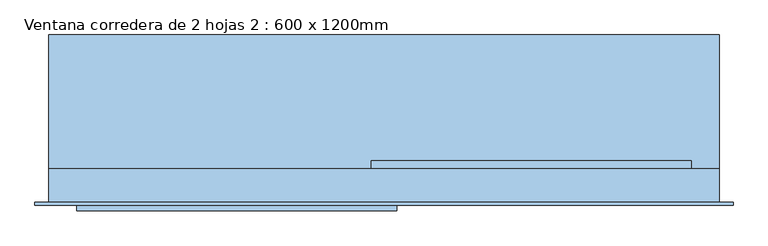
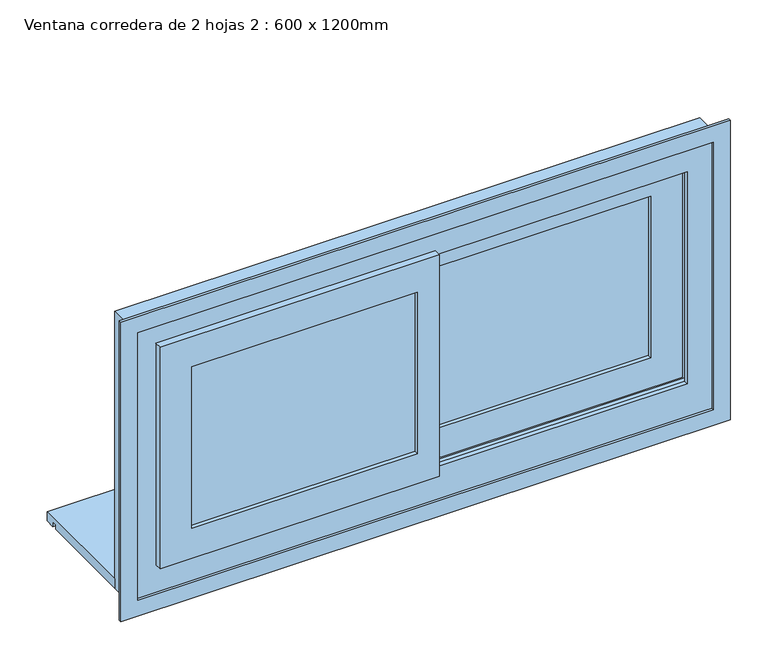
"""IFC4 building model written with IfcOpenShell, lengths in millimetres: window geometry, Ventana corredera de 2 hojas 2 : 600 x 1200mm."""

from ifc_helpers import new_model, si_unit, frame, origin, place, context, project, spatial, polyline, outline, extrude, faceted_brep, source, transform, mapped, element, save


def ventana_corredera_de_2_hojas_2_600_x_1200mm_91e0f78e(model_context):
    return source(origin(), model_context, "Body", "SolidModel", [
        extrude(outline(polyline([(225.0, 920.0), (225.0, 900.0), (205.0, 900.0), (205.0, 910.0), (195.0, 910.0), (195.0, 900.0), (-15.0, 900.0), (-15.0, 920.0), (225.0, 920.0)])), frame((-600.0, 0.0, 0.0), z_axis=(1.0, 0.0, 0.0), x_axis=(0.0, 1.0, 0.0)), (0.0, 0.0, 1.0), 1200.0),
        faceted_brep([(22.5, -90.0, 970.0011599), (22.5, -75.0, 970.0011599), (22.5, -75.0, 990.0011599), (22.5, -65.0, 990.0011599), (22.5, -65.0, 970.0011599), (22.5, -42.0, 970.0011599), (22.5, -42.0, 1449.9988401), (22.5, -65.0, 1449.9988401), (22.5, -65.0, 1429.9988401), (22.5, -75.0, 1429.9988401), (22.5, -75.0, 1449.9988401), (22.5, -90.0, 1449.9988401), (-549.9988401, -90.0, 970.0011599), (-549.9988401, -75.0, 970.0011599), (-549.9988401, -75.0, 1449.9988401), (-529.9988401, -75.0, 1429.9988401), (-529.9988401, -75.0, 990.0011599), (-529.9988401, -65.0, 990.0011599), (-529.9988401, -65.0, 1429.9988401), (-549.9988401, -65.0, 1449.9988401), (-549.9988401, -65.0, 970.0011599), (-549.9988401, -50.0, 970.0011599), (0.0, -50.0, 970.0011599), (0.0, -42.0, 970.0011599), (0.0, -42.0, 1449.9988401), (-549.9988401, -90.0, 1449.9988401), (-484.9988401, -90.0, 1035.0011599), (-484.9988401, -90.0, 1384.9988401), (-22.5, -90.0, 1384.9988401), (-22.5, -90.0, 1035.0011599), (-549.9988401, -50.0, 1449.9988401), (0.0, -50.0, 1449.9988401), (-484.9988401, -50.0, 1384.9988401), (-484.9988401, -50.0, 1035.0011599), (-22.5, -50.0, 1035.0011599), (-22.5, -50.0, 1384.9988401), (-484.9988401, -58.0, 1384.9988401), (-484.9988401, -58.0, 1035.0011599), (-22.5, -58.0, 1035.0011599), (-22.5, -58.0, 1384.9988401), (-484.9988401, -82.0, 1035.0011599), (-484.9988401, -82.0, 1384.9988401), (-22.5, -82.0, 1384.9988401), (-22.5, -82.0, 1035.0011599), (-504.9988401, -82.0, 1015.0011599), (-504.9988401, -82.0, 1404.9988401), (-2.5, -82.0, 1404.9988401), (-2.5, -82.0, 1015.0011599), (-504.9988401, -58.0, 1015.0011599), (-504.9988401, -58.0, 1404.9988401), (-2.5, -58.0, 1015.0011599), (-2.5, -58.0, 1404.9988401)], [[[0, 1, 2, 3, 4, 5, 6, 7, 8, 9, 10, 11]], [[1, 0, 12, 13]], [[2, 1, 13, 14, 10, 9, 15, 16]], [[3, 2, 16, 17]], [[4, 3, 17, 18, 8, 7, 19, 20]], [[5, 4, 20, 21, 22, 23]], [[6, 5, 23, 24]], [[12, 0, 11, 25], [26, 27, 28, 29]], [[21, 30, 31, 22], [32, 33, 34, 35]], [[30, 21, 20, 19]], [[24, 23, 22, 31]], [[33, 32, 36, 37]], [[33, 37, 38, 34]], [[38, 39, 35, 34]], [[18, 17, 16, 15]], [[14, 13, 12, 25]], [[27, 26, 40, 41]], [[29, 28, 42, 43]], [[40, 26, 29, 43]], [[44, 45, 46, 47], [41, 40, 43, 42]], [[45, 44, 48, 49]], [[50, 47, 46, 51]], [[48, 44, 47, 50]], [[49, 48, 50, 51], [37, 36, 39, 38]], [[19, 7, 6, 24, 31, 30]], [[8, 18, 15, 9]], [[10, 14, 25, 11]], [[36, 32, 35, 39]], [[27, 41, 42, 28]], [[45, 49, 51, 46]]]),
        faceted_brep([(-22.5, 0.0, 1449.9988401), (549.9988401, 0.0, 1449.9988401), (549.9988401, 0.0, 970.0011599), (-22.5, 0.0, 970.0011599), (484.9988401, 0.0, 1035.0011599), (484.9988401, 0.0, 1384.9988401), (22.5, 0.0, 1384.9988401), (22.5, 0.0, 1035.0011599), (549.9988401, -15.0, 1449.9988401), (549.9988401, -15.0, 970.0011599), (-22.5, -15.0, 970.0011599), (-22.5, -25.0, 1449.9988401), (-22.5, -25.0, 1429.9988401), (-22.5, -15.0, 1429.9988401), (-22.5, -15.0, 1449.9988401), (-22.5, -15.0, 990.0011599), (-22.5, -25.0, 990.0011599), (-22.5, -25.0, 970.0011599), (-22.5, -48.0, 970.0011599), (-22.5, -48.0, 1449.9988401), (484.9988401, -8.0, 1035.0011599), (484.9988401, -8.0, 1384.9988401), (22.5, -8.0, 1384.9988401), (22.5, -8.0, 1035.0011599), (529.9988401, -15.0, 1429.9988401), (529.9988401, -15.0, 990.0011599), (529.9988401, -25.0, 990.0011599), (549.9988401, -25.0, 1449.9988401), (549.9988401, -25.0, 970.0011599), (529.9988401, -25.0, 1429.9988401), (549.9988401, -40.0, 970.0011599), (0.0, -40.0, 970.0011599), (0.0, -48.0, 970.0011599), (0.0, -48.0, 1449.9988401), (0.0, -40.0, 1449.9988401), (549.9988401, -40.0, 1449.9988401), (484.9988401, -40.0, 1384.9988401), (484.9988401, -40.0, 1035.0011599), (22.5, -40.0, 1035.0011599), (22.5, -40.0, 1384.9988401), (484.9988401, -32.0, 1384.9988401), (484.9988401, -32.0, 1035.0011599), (22.5, -32.0, 1035.0011599), (22.5, -32.0, 1384.9988401), (504.9988401, -32.0, 1404.9988401), (504.9988401, -32.0, 1015.0011599), (2.5, -32.0, 1015.0011599), (2.5, -32.0, 1404.9988401), (504.9988401, -8.0, 1404.9988401), (504.9988401, -8.0, 1015.0011599), (2.5, -8.0, 1015.0011599), (2.5, -8.0, 1404.9988401)], [[[0, 1, 2, 3], [4, 5, 6, 7]], [[8, 9, 2, 1]], [[9, 10, 3, 2]], [[11, 12, 13, 14, 0, 3, 10, 15, 16, 17, 18, 19]], [[5, 4, 20, 21]], [[7, 6, 22, 23]], [[20, 4, 7, 23]], [[14, 13, 24, 25, 15, 10, 9, 8]], [[26, 16, 15, 25]], [[12, 11, 27, 28, 17, 16, 26, 29]], [[18, 17, 28, 30, 31, 32]], [[19, 18, 32, 33]], [[33, 32, 31, 34]], [[30, 35, 34, 31], [36, 37, 38, 39]], [[37, 36, 40, 41]], [[37, 41, 42, 38]], [[39, 38, 42, 43]], [[35, 30, 28, 27]], [[44, 45, 46, 47], [41, 40, 43, 42]], [[48, 49, 45, 44]], [[45, 49, 50, 46]], [[51, 47, 46, 50]], [[49, 48, 51, 50], [21, 20, 23, 22]], [[29, 26, 25, 24]], [[0, 14, 8, 1]], [[5, 21, 22, 6]], [[13, 12, 29, 24]], [[11, 19, 33, 34, 35, 27]], [[40, 36, 39, 43]], [[48, 44, 47, 51]]]),
        extrude(outline(polyline([(-7.5, -58.0), (-7.5, -82.0), (-499.9988401, -82.0), (-499.9988401, -58.0), (-7.5, -58.0)])), frame((0.0, 0.0, 1020.0011599), z_axis=(0.0, 0.0, 1.0), x_axis=(1.0, 0.0, 0.0)), (0.0, 0.0, 1.0), 379.9976801),
        extrude(outline(polyline([(499.9988401, -8.0), (499.9988401, -32.0), (7.5, -32.0), (7.5, -8.0), (499.9988401, -8.0)])), frame((0.0, 0.0, 1020.0011599), z_axis=(0.0, 0.0, 1.0), x_axis=(1.0, 0.0, 0.0)), (0.0, 0.0, 1.0), 379.9976801),
        faceted_brep([(600.0, -15.0, 1500.0), (600.0, -75.0, 1500.0), (600.0, -75.0, 900.0), (600.0, -15.0, 900.0), (-600.0, -75.0, 1500.0), (-600.0, -75.0, 900.0), (-539.9988401, -75.0, 1439.9988401), (539.9988401, -75.0, 1439.9988401), (539.9988401, -75.0, 980.0011599), (-539.9988401, -75.0, 980.0011599), (-600.0, -15.0, 900.0), (-600.0, -15.0, 1500.0), (539.9988401, -15.0, 1439.9988401), (-539.9988401, -15.0, 1439.9988401), (-539.9988401, -15.0, 980.0011599), (539.9988401, -15.0, 980.0011599), (539.9988401, -25.0, 1439.9988401), (539.9988401, -25.0, 980.0011599), (-539.9988401, -25.0, 980.0011599), (564.9988401, -25.0, 1464.9988401), (-564.9988401, -25.0, 1464.9988401), (-564.9988401, -25.0, 955.0011599), (564.9988401, -25.0, 955.0011599), (-539.9988401, -25.0, 1439.9988401), (564.9988401, -65.0, 1464.9988401), (564.9988401, -65.0, 955.0011599), (-564.9988401, -65.0, 955.0011599), (-564.9988401, -65.0, 1464.9988401), (539.9988401, -65.0, 1439.9988401), (-539.9988401, -65.0, 1439.9988401), (-539.9988401, -65.0, 980.0011599), (539.9988401, -65.0, 980.0011599)], [[[0, 1, 2, 3]], [[2, 1, 4, 5], [6, 7, 8, 9]], [[3, 2, 5, 10]], [[10, 11, 0, 3], [12, 13, 14, 15]], [[16, 12, 15, 17]], [[17, 15, 14, 18]], [[19, 20, 21, 22], [23, 16, 17, 18]], [[24, 19, 22, 25]], [[25, 22, 21, 26]], [[27, 24, 25, 26], [28, 29, 30, 31]], [[7, 28, 31, 8]], [[8, 31, 30, 9]], [[13, 23, 18, 14]], [[20, 27, 26, 21]], [[29, 6, 9, 30]], [[4, 11, 10, 5]], [[11, 4, 1, 0]], [[23, 13, 12, 16]], [[27, 20, 19, 24]], [[6, 29, 28, 7]]]),
        extrude(outline(polyline([(1525.0, -625.0), (875.0, -625.0), (875.0, 625.0), (1525.0, 625.0), (1525.0, -625.0)]), holes=[polyline([(1490.0, 590.0), (910.0, 590.0), (910.0, -590.0), (1490.0, -590.0), (1490.0, 590.0)])]), frame((0.0, -80.0, 0.0), z_axis=(0.0, 1.0, 0.0), x_axis=(0.0, 0.0, 1.0)), (0.0, 0.0, 1.0), 5.0),
    ])


if __name__ == "__main__":
    model = new_model("IFC4")
    model_context = context("Model", 3, world=origin())
    ifc_project = project(units=[si_unit("LENGTHUNIT", "METRE", prefix="MILLI")], contexts=[model_context])
    site = spatial("IfcSite", under=ifc_project)
    building = spatial("IfcBuilding", under=site)
    placement = place(None, origin())
    ventana_corredera_de_2_hojas_2_600_x_1200mm_shape = ventana_corredera_de_2_hojas_2_600_x_1200mm_91e0f78e(model_context)
    element("IfcWindow", 1, ObjectType="Ventana corredera de 2 hojas 2 : 600 x 1200mm", at=placement, inside=building, context=model_context, shape_type="MappedRepresentation", body=[
        mapped(ventana_corredera_de_2_hojas_2_600_x_1200mm_shape, transform((0.0, 0.0, 0.0), x_axis=(1.0, 0.0, 0.0), y_axis=(0.0, 1.0, 0.0), z_axis=(0.0, 0.0, 1.0))),
    ])
    save(model, "model.ifc")

# Revit data of these elements
# Type "Ventana corredera de 2 hojas 2 : 600 x 1200mm"
#   Type Mark = "48"
#   Construction Type Id = "GSP4R"
#   Analytic Construction = "1/8 en cristalera simple Pilkington"
#   Grosor de pared [instance default] = 0.20 m
#   Visual Light Transmittance = 0.9
#   Anchura de cubrejuntas = 0.035 m
#   Grosor de cubrejuntas = 0.005 m
#   Solar Heat Gain Coefficient = 0.78
#   Grosor de antepecho = 0.02 m
#   Profundidad de antepecho [instance default] = 0.29 m
#   Rough Width = 1.20 m
#   Rough Height = 0.60 m
#   Anchura de marco de panel = 0.065 m
#   Anchura de marco de panel intermedio = 0.045 m
#   Height = 0.60 m
#   Heat Transfer Coefficient (U) = 3.6886 W/(m²·K)
#   Anchura de marco = 0.060001 m
#   Grosor de marco = 0.06 m
#   Distancia entre antepecho y muro = 0.15 m
#   Altura de antepecho por defecto = 0.90 m
#   Width = 1.20 m
#   Define Thermal Properties by = 1
#   Material de antepecho = none
#   Material de cristalera = Vidrio
#   Material de estructura = none
#   Wall Closure = (empty or 0)
# Element 1 (IfcWindow, "Ventana corredera de 2 hojas 2 : 600 x 1200mm")
#   Grosor de pared = 0.15 m
#   Profundidad de antepecho = 0.24 m
#   Materials on its faces: "Vidrio", "Madera - Tinte"
# Materials
#   "Vidrio": class "Vidrio", colour RGB 245 245 243, transparency 1, Description = "Vidrio de cal sodada", Cost = 0
#   "Madera - Tinte": class "Madera", colour RGB 173 132 96, transparency 0, Cost = 0
